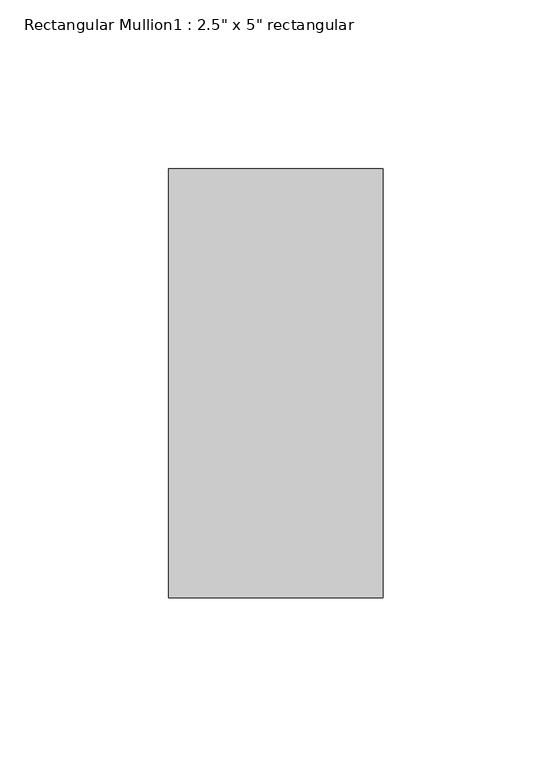
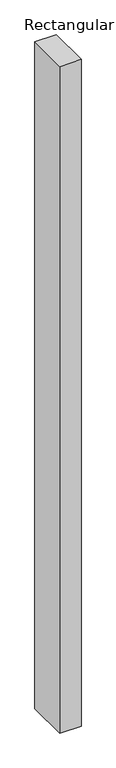
"""IFC4 building model written with IfcOpenShell, lengths in millimetres: member geometry."""

from ifc_helpers import new_model, si_unit, frame, origin, place, context, project, spatial, polyline, outline, extrude, source, transform, mapped, element, save


def member_a50b3385(model_context):
    return source(origin(), model_context, "Body", "SweptSolid", [
        extrude(outline(polyline([(31.75, 63.5), (31.75, -63.5), (-31.75, -63.5), (-31.75, 63.5), (31.75, 63.5)])), frame((0.0, 0.0, -2091.69), z_axis=(0.0, 0.0, 1.0), x_axis=(1.0, 0.0, 0.0)), (0.0, 0.0, 1.0), 2091.69),
    ])


if __name__ == "__main__":
    model = new_model("IFC4")
    model_context = context("Model", 3, world=origin())
    ifc_project = project(units=[si_unit("LENGTHUNIT", "METRE", prefix="MILLI")], contexts=[model_context])
    site = spatial("IfcSite", under=ifc_project)
    building = spatial("IfcBuilding", under=site)
    placement = place(None, origin())
    member_shape = member_a50b3385(model_context)
    element("IfcMember", 1, ObjectType="Rectangular Mullion1 : 2.5\" x 5\" rectangular", at=placement, inside=building, context=model_context, shape_type="MappedRepresentation", body=[
        mapped(member_shape, transform((0.0, 0.0, 0.0), x_axis=(1.0, 0.0, 0.0), y_axis=(0.0, 1.0, 0.0), z_axis=(0.0, 0.0, 1.0))),
    ])
    save(model, "model.ifc")

# Revit data of these elements
# Type "Rectangular Mullion1 : 2.5\" x 5\" rectangular"
#   built-in parameter 1007304 = 0.416667 (stored number, unit not read)
#   built-in parameter 1007301 = 0.104167 (stored number, unit not read)
#   built-in parameter 1007300 = 0.104167 (stored number, unit not read)
# Element 1 (IfcMember, "Rectangular Mullion1 : 2.5\" x 5\" rectangular")
#   Materials on its faces: "support-frame"
# Materials
#   "support-frame": class "Unassigned", colour RGB 233 233 233, transparency 0, Cost = 0
